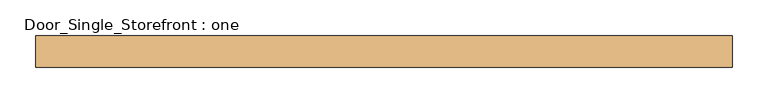
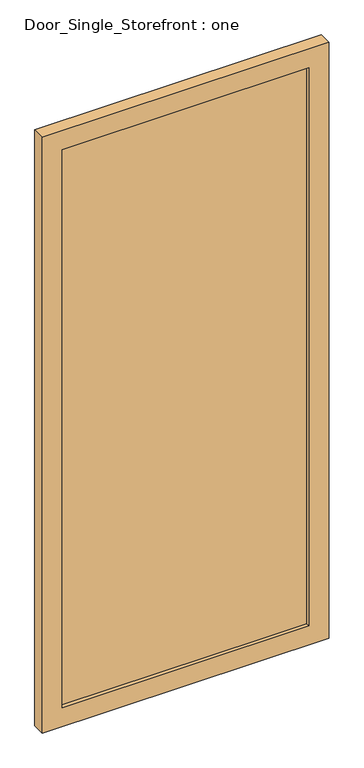
"""IFC4 building model written with IfcOpenShell, lengths in millimetres: door geometry, Door_Single_Storefront : one."""

from ifc_helpers import new_model, si_unit, frame, origin, place, context, project, spatial, polyline, outline, extrude, source, transform, mapped, element, save


def door_single_storefront_one_ee7034be(model_context):
    return source(origin(), model_context, "Body", "SweptSolid", [
        extrude(outline(polyline([(421.878125, 6.35), (421.878125, -12.7), (-421.878125, -12.7), (-421.878125, 6.35), (421.878125, 6.35)])), frame((0.0, 0.0, 68.2625), z_axis=(0.0, 0.0, 1.0), x_axis=(1.0, 0.0, 0.0)), (0.0, 0.0, 1.0), 2016.125),
        extrude(outline(polyline([(2152.65, -490.140625), (0.0, -490.140625), (0.0, 490.140625), (2152.65, 490.140625), (2152.65, -490.140625)]), holes=[polyline([(68.2625, 421.878125), (68.2625, -421.878125), (2084.3875, -421.878125), (2084.3875, 421.878125), (68.2625, 421.878125)])]), frame((0.0, -25.4, 0.0), z_axis=(0.0, 1.0, 0.0), x_axis=(0.0, 0.0, 1.0)), (0.0, 0.0, 1.0), 44.45),
    ])


if __name__ == "__main__":
    model = new_model("IFC4")
    model_context = context("Model", 3, world=origin())
    ifc_project = project(units=[si_unit("LENGTHUNIT", "METRE", prefix="MILLI")], contexts=[model_context])
    site = spatial("IfcSite", under=ifc_project)
    building = spatial("IfcBuilding", under=site)
    placement = place(None, origin())
    door_single_storefront_one_shape = door_single_storefront_one_ee7034be(model_context)
    element("IfcDoor", 1, ObjectType="Door_Single_Storefront : one", at=placement, inside=building, context=model_context, shape_type="MappedRepresentation", body=[
        mapped(door_single_storefront_one_shape, transform((0.0, 0.0, 0.0), x_axis=(1.0, 0.0, 0.0), y_axis=(0.0, 1.0, 0.0), z_axis=(0.0, 0.0, 1.0))),
    ])
    save(model, "model.ifc")

# Revit data of these elements
# Type "Door_Single_Storefront : one"
#   Type Mark = "29"
#   OD_DS_Door_Material = "ALUM./GLAZING"
#   OD_DS_Door_Type = "STOREFRONT (NARROW STILE)"
#   OD_DS_Lockset = "ENTRY LOCK (INSIDE ADA LEVER ALWAYS ACTIVE)"
#   Analytic Construction = "<None>"
#   angle open [instance default] = 132.952°
#   Stile_Width = 0' - 2 11/16"
#   Door_Thickness = 0' - 1 3/4"
#   Door_Offset = 0' - 1"
#   Glass_Material = TEMPERED INSULATED GLAZING (CARDINAL GLASS LoĒ²-240\nOR EQUIVALENT)
#   Frame_Material = KAWNEER 260 INSULCLADTM THERMAL ENTRANCE - CLEAR ANODIZED ALUM.
#   Function = (empty or 0)
# Element 1 (IfcDoor, "Door_Single_Storefront : one")
#   angle open = 170.00°
#   Materials on its faces: "KAWNEER 260 INSULCLADTM THERMAL ENTRANCE - CLEAR ANODIZED ALUM.", "TEMPERED INSULATED GLAZING (CARDINAL GLASS LoĒ²-240\nOR EQUIVALENT)"
# Materials
#   "TEMPERED INSULATED GLAZING (CARDINAL GLASS LoĒ²-240\nOR EQUIVALENT)": class "Glass", colour RGB 196 205 210, transparency 0.85, Description = "Soda Lime Glass", Cost = 0
#   "KAWNEER 260 INSULCLADTM THERMAL ENTRANCE - CLEAR ANODIZED ALUM.": class "Metal", colour RGB 244 244 244, transparency 0, Description = "Aluminum 6061", Cost = 0
